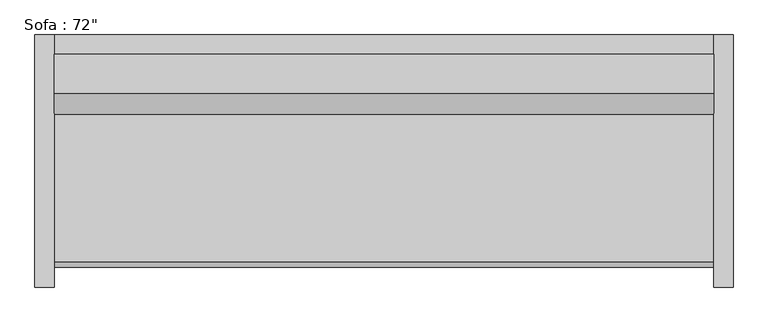
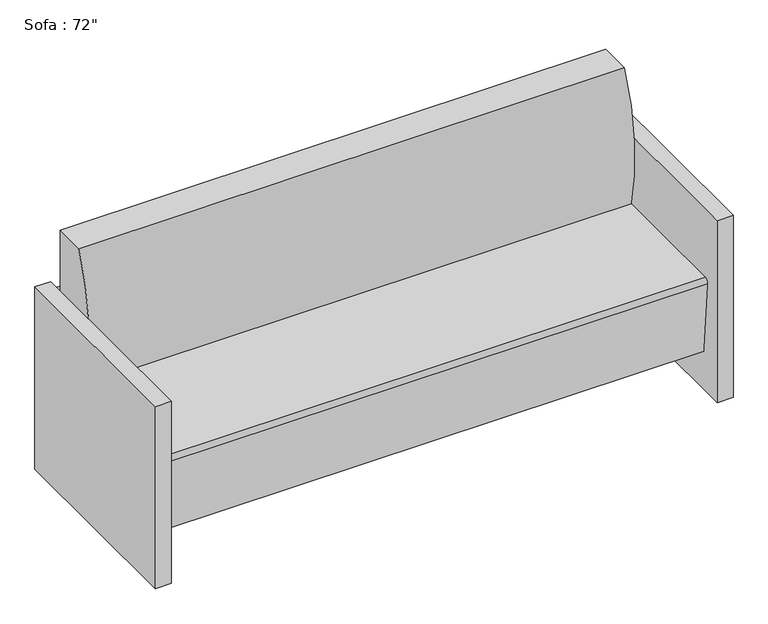
"""IFC4 building model written with IfcOpenShell, lengths in millimetres: furniture geometry."""

from ifc_helpers import new_model, si_unit, point, frame, frame_2d, origin, origin_with_axes, place, context, project, spatial, polyline, circle_curve, trimmed, segment, composite_curve, outline, extrude, source, transform, mapped, element, save


def furniture_a4ffab56(model_context):
    return source(origin(), model_context, "Body", "SweptSolid", [
        extrude(outline(polyline([(-793.2295082, 425.5540984), (-793.2295082, 476.3540984), (933.9704918, 476.3540984), (933.9704918, 425.5540984), (-793.2295082, 425.5540984)])), frame((0.0, 0.0, 457.2), z_axis=(0.0, 0.0, 1.0), x_axis=(1.0, 0.0, 0.0)), (0.0, 0.0, 1.0), 127.0),
        extrude(outline(polyline([(-793.2295082, 425.5540984), (-793.2295082, 476.3540984), (933.9704918, 476.3540984), (933.9704918, 425.5540984), (-793.2295082, 425.5540984)])), frame((0.0, 0.0, 266.7), z_axis=(0.0, 0.0, 1.0), x_axis=(1.0, 0.0, 0.0)), (0.0, 0.0, 1.0), 127.0),
        extrude(outline(polyline([(-793.2295082, 425.5540984), (-793.2295082, 476.3540984), (933.9704918, 476.3540984), (933.9704918, 425.5540984), (-793.2295082, 425.5540984)])), frame((0.0, 0.0, 76.2), z_axis=(0.0, 0.0, 1.0), x_axis=(1.0, 0.0, 0.0)), (0.0, 0.0, 1.0), 127.0),
        extrude(outline(composite_curve([segment(trimmed(circle_curve(frame_2d((926.517198, 542.5300036)), 660.4), [point((286.1764935, 381.0))], [point((323.9540984, 812.8))], False, "CARTESIAN"), True, "CONTINUOUS"), segment(polyline([(323.9540984, 812.8), (425.5540984, 812.8), (425.5540984, 127.9665467), (-111.108343, 127.9665467), (-132.0379563, 367.1931221)]), True, "CONTINUOUS"), segment(trimmed(circle_curve(frame_2d((-119.3862837, 368.3)), 12.7), [point((-132.0379563, 367.1931221))], [point((-119.3862837, 381.0))], False, "CARTESIAN"), True, "CONTINUOUS"), segment(polyline([(-119.3862837, 381.0), (286.1764935, 381.0)]), True, "CONTINUOUS")], self_intersect=False)), frame((-793.2295082, 0.0, 0.0), z_axis=(1.0, 0.0, 0.0), x_axis=(0.0, 1.0, 0.0)), (0.0, 0.0, 1.0), 1727.2),
        extrude(outline(polyline([(-844.0295082, 476.3540984), (-793.2295082, 476.3540984), (-793.2295082, -184.0459016), (-844.0295082, -184.0459016), (-844.0295082, 476.3540984)])), origin_with_axes(), (0.0, 0.0, 1.0), 609.6),
        extrude(outline(polyline([(984.7704918, 476.3540984), (984.7704918, -184.0459016), (933.9704918, -184.0459016), (933.9704918, 476.3540984), (984.7704918, 476.3540984)])), origin_with_axes(), (0.0, 0.0, 1.0), 609.6),
    ])


if __name__ == "__main__":
    model = new_model("IFC4")
    model_context = context("Model", 3, world=origin())
    ifc_project = project(units=[si_unit("LENGTHUNIT", "METRE", prefix="MILLI")], contexts=[model_context])
    site = spatial("IfcSite", under=ifc_project)
    building = spatial("IfcBuilding", under=site)
    placement = place(None, origin())
    furniture_shape = furniture_a4ffab56(model_context)
    element("IfcFurniture", 1, ObjectType="Sofa : 72\"", at=placement, inside=building, context=model_context, shape_type="MappedRepresentation", body=[
        mapped(furniture_shape, transform((0.0, 0.0, 0.0), x_axis=(1.0, 0.0, 0.0), y_axis=(0.0, 1.0, 0.0), z_axis=(0.0, 0.0, 1.0))),
    ])
    save(model, "model.ifc")

# Revit data of these elements
# Type "Sofa : 72\""
#   Assembly Code = "E2020200"
#   Width = 6' - 0"
#   Seat Material = Linen, Beige
#   Frame Material = Cherry
#   Default Elevation = 0
# Element 1 (IfcFurniture, "Sofa : 72\"")
#   Materials on its faces: "Cherry", "Linen, Beige"
# Materials
#   "Linen, Beige": class "Textile", colour RGB 199 194 175, transparency 0, Description = "Linen, beige", Cost = 0
#   "Cherry": class "Wood", colour RGB 233 182 144, transparency 0, Description = "Prunus Serotina", Cost = 0
